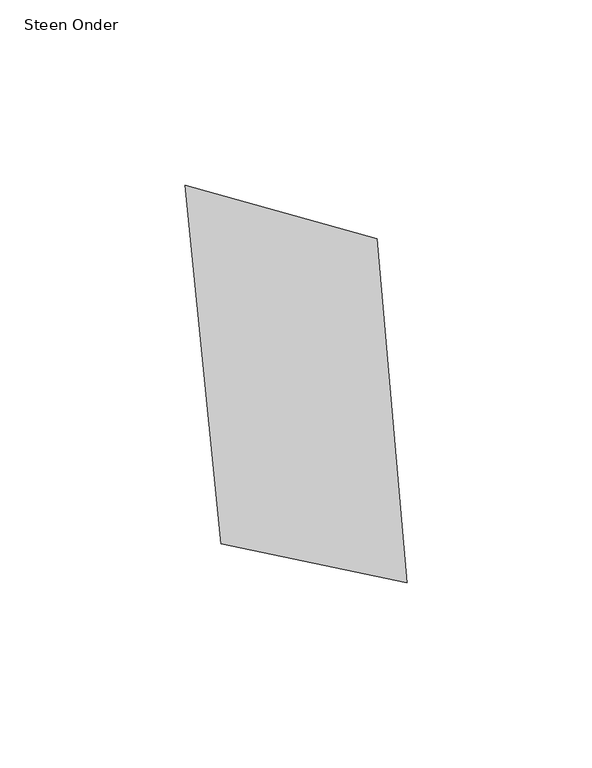
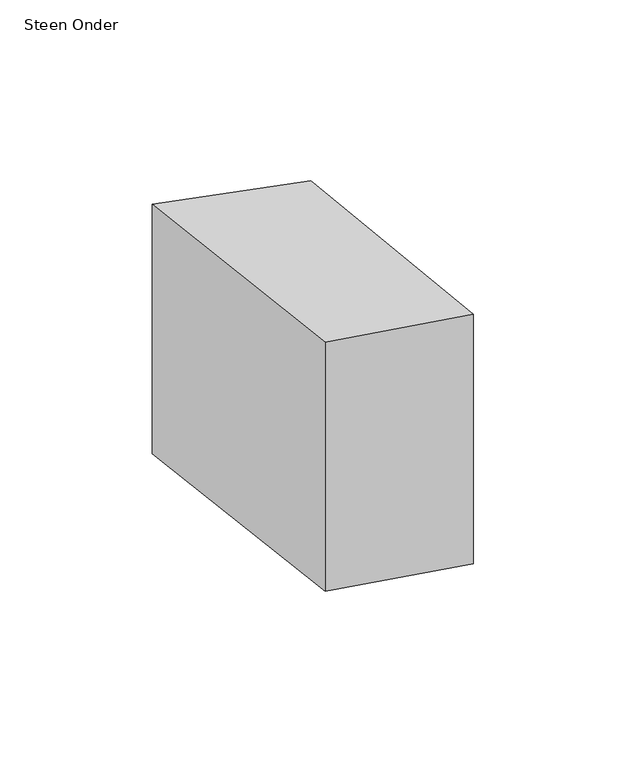
"""IFC4 building model written with IfcOpenShell, lengths in millimetres: proxy geometry, 00_GMA_steen_versie_4 : Steen Onder."""

import ifcopenshell
import ifcopenshell.guid

model = None  # the IFC model being written
_history = None  # IfcOwnerHistory: only IFC2X3 demands one
_inside = {}  # id of a spatial element -> (the spatial element, [elements in it])
_under = {}  # id of a project, library or spatial element -> (it, [spatial elements below it])
_declared = {}  # id of a project -> (the project, [libraries it declares])
_typed = {}  # id of a type object -> (the type object, [elements of that type])
_made_of = {}  # id of a material, layer set ... -> (it, [elements and type objects made of it])


def new_model(schema):
    """Start an empty IFC model of exactly this schema.

    Asked for "IFC4X3", IfcOpenShell would pick the latest addendum, in which some entities
    have other attributes; the version numbers below select the first issue.
    IFC2X3 requires an IfcOwnerHistory on every rooted entity: one is made here for all.
    """
    global model, _history
    if schema == "IFC4X3":
        model = ifcopenshell.file(schema_version=(4, 3, 0, 0))
    else:
        model = ifcopenshell.file(schema=schema)
    _inside.clear()
    _under.clear()
    _declared.clear()
    _typed.clear()
    _made_of.clear()
    _history = None
    if model.schema == "IFC2X3":
        org = make("IfcOrganization", Name="unknown")
        user = make(
            "IfcPersonAndOrganization",
            ThePerson=make("IfcPerson", FamilyName="unknown"),
            TheOrganization=org,
        )
        app = make(
            "IfcApplication",
            ApplicationDeveloper=org,
            Version="unknown",
            ApplicationFullName="unknown",
            ApplicationIdentifier="unknown",
        )
        _history = make(
            "IfcOwnerHistory",
            OwningUser=user,
            OwningApplication=app,
            ChangeAction="ADDED",
            CreationDate=0,
        )
    return model


def make(cls, **values):
    """One entity of the class cls with the attributes given. An attribute that is None is left unset."""
    return model.create_entity(
        cls, **{name: value for name, value in values.items() if value is not None}
    )


def rooted(cls, **values):
    """An entity with a GlobalId (a new one), such as an element, a storey or a relation."""
    return make(cls, GlobalId=ifcopenshell.guid.new(), OwnerHistory=_history, **values)


def si_unit(unit_type, name, prefix=None):
    """IfcSIUnit, for example si_unit("LENGTHUNIT", "METRE", prefix="MILLI")."""
    return make("IfcSIUnit", UnitType=unit_type, Prefix=prefix, Name=name)


def assignment(units):
    """IfcUnitAssignment: the units of a project."""
    return None if units is None else make("IfcUnitAssignment", Units=units)


def point(xyz):
    """IfcCartesianPoint."""
    return None if xyz is None else make("IfcCartesianPoint", Coordinates=xyz)


def direction(xyz):
    """IfcDirection."""
    return None if xyz is None else make("IfcDirection", DirectionRatios=xyz)


def frame(location, z_axis=None, x_axis=None):
    """IfcAxis2Placement3D, a coordinate frame: its origin and axes. An axis left out is left unset."""
    return make(
        "IfcAxis2Placement3D",
        Location=point(location),
        Axis=direction(z_axis),
        RefDirection=direction(x_axis),
    )


def origin():
    """The frame at (0, 0, 0) with its axes left unset."""
    return frame((0.0, 0.0, 0.0))


def origin_with_axes():
    """The frame at (0, 0, 0) with the z axis (0, 0, 1) and the x axis (1, 0, 0) written out."""
    return frame((0.0, 0.0, 0.0), z_axis=(0.0, 0.0, 1.0), x_axis=(1.0, 0.0, 0.0))


def place(relative_to, where):
    """IfcLocalPlacement: puts the frame where relative to a parent placement (None: the world)."""
    return make(
        "IfcLocalPlacement", PlacementRelTo=relative_to, RelativePlacement=where
    )


def context(
    kind, dimensions, precision=None, world=None, true_north=None, identifier=None
):
    """IfcGeometricRepresentationContext, for example the 3D "Model" context."""
    return make(
        "IfcGeometricRepresentationContext",
        ContextIdentifier=identifier,
        ContextType=kind,
        CoordinateSpaceDimension=dimensions,
        Precision=precision,
        WorldCoordinateSystem=world,
        TrueNorth=true_north,
    )


def project(units=None, contexts=None):
    """IfcProject with its units and contexts."""
    return rooted(
        "IfcProject",
        Name="project",
        RepresentationContexts=contexts,
        UnitsInContext=assignment(units),
    )


def spatial(cls, under=None, at=None, **own):
    """A site, building, storey or space (cls), placed at a placement, below another one or the project."""
    s = rooted(cls, ObjectPlacement=at, **own)
    if under is not None:
        _under.setdefault(under.id(), (under, []))[1].append(s)
    return s


def polyline(points):
    """IfcPolyline through the points."""
    return make("IfcPolyline", Points=[point(p) for p in points])


def outline(outer, holes=None, kind="AREA"):
    """IfcArbitraryClosedProfileDef: a profile drawn as a closed curve; with holes, ...WithVoids."""
    if holes is None:
        return make("IfcArbitraryClosedProfileDef", ProfileType=kind, OuterCurve=outer)
    return make(
        "IfcArbitraryProfileDefWithVoids",
        ProfileType=kind,
        OuterCurve=outer,
        InnerCurves=holes,
    )


def extrude(swept, where, along, depth):
    """IfcExtrudedAreaSolid: the profile swept, set in the frame where, extruded along a direction by depth."""
    return make(
        "IfcExtrudedAreaSolid",
        SweptArea=swept,
        Position=where,
        ExtrudedDirection=direction(along),
        Depth=depth,
    )


def shape(context_of_items, identifier, shape_type, items):
    """IfcShapeRepresentation: the items that make up one representation, for example the "Body"."""
    return make(
        "IfcShapeRepresentation",
        ContextOfItems=context_of_items,
        RepresentationIdentifier=identifier,
        RepresentationType=shape_type,
        Items=items,
    )


def source(mapping_origin, context_of_items, identifier, shape_type, items):
    """IfcRepresentationMap: a shape defined once, which mapped items show again and again."""
    return make(
        "IfcRepresentationMap",
        MappingOrigin=mapping_origin,
        MappedRepresentation=shape(context_of_items, identifier, shape_type, items),
    )


def transform(
    local_origin,
    x_axis=None,
    y_axis=None,
    z_axis=None,
    scale=None,
    scale2=None,
    scale3=None,
    uniform=True,
):
    """IfcCartesianTransformationOperator3D, or its non-uniform kind. x_axis, y_axis, z_axis: its Axis1, 2, 3."""
    if uniform:
        return make(
            "IfcCartesianTransformationOperator3D",
            Axis1=direction(x_axis),
            Axis2=direction(y_axis),
            LocalOrigin=point(local_origin),
            Scale=scale,
            Axis3=direction(z_axis),
        )
    return make(
        "IfcCartesianTransformationOperator3DnonUniform",
        Axis1=direction(x_axis),
        Axis2=direction(y_axis),
        LocalOrigin=point(local_origin),
        Scale=scale,
        Axis3=direction(z_axis),
        Scale2=scale2,
        Scale3=scale3,
    )


def mapped(mapping_source, mapping_target):
    """IfcMappedItem: shows the shape of a source again, moved by a transform."""
    return make(
        "IfcMappedItem", MappingSource=mapping_source, MappingTarget=mapping_target
    )


def made_of(thing, what):
    """Note that an element or type object is made of a material, layer set ...; save() writes the relation."""
    if what is not None:
        _made_of.setdefault(what.id(), (what, []))[1].append(thing)
    return thing


def element(
    cls,
    number,
    at=None,
    inside=None,
    cuts=None,
    type_object=None,
    material=None,
    context=None,
    identifier="Body",
    shape_type=None,
    held_by="IfcProductDefinitionShape",
    body=None,
    shapes=None,
    **own,
):
    """One element of the class cls, such as IfcWall. Its Tag is "e" and its number.

    at: its placement. inside: the storey or other place that contains it. cuts: it is an
    opening in that element (IfcRelVoidsElement). A single representation is given by context,
    identifier, shape_type and body (its items); several are given by shapes. held_by: the class
    of the entity that holds the representations. save() writes the other relations.
    """
    e = rooted(cls, Tag="e%d" % number, ObjectPlacement=at, **own)
    if body is not None:
        shapes = [shape(context, identifier, shape_type, body)]
    if shapes is not None:
        e.Representation = make(held_by, Representations=shapes)
    if inside is not None:
        _inside.setdefault(inside.id(), (inside, []))[1].append(e)
    if cuts is not None:
        rooted(
            "IfcRelVoidsElement", RelatingBuildingElement=cuts, RelatedOpeningElement=e
        )
    if type_object is not None:
        _typed.setdefault(type_object.id(), (type_object, []))[1].append(e)
    return made_of(e, material)


def aggregate(whole, parts):
    """IfcRelAggregates: a whole, such as a stair, and the parts it consists of."""
    return rooted("IfcRelAggregates", RelatingObject=whole, RelatedObjects=parts)


def save(model, path):
    """Write the relations noted so far, then the file.

    IfcRelAggregates (storeys below a building ...), IfcRelContainedInSpatialStructure (elements
    in a storey), IfcRelDefinesByType, IfcRelAssociatesMaterial and IfcRelDeclares: one each for
    every whole, place, type object, material and project.
    """
    for whole, parts in _under.values():
        aggregate(whole, parts)
    for where, things in _inside.values():
        rooted(
            "IfcRelContainedInSpatialStructure",
            RelatedElements=things,
            RelatingStructure=where,
        )
    for kind, things in _typed.values():
        rooted("IfcRelDefinesByType", RelatedObjects=things, RelatingType=kind)
    for what, things in _made_of.values():
        rooted("IfcRelAssociatesMaterial", RelatedObjects=things, RelatingMaterial=what)
    for by, libraries in _declared.values():
        rooted("IfcRelDeclares", RelatingContext=by, RelatedDefinitions=libraries)
    model.write(path)


def steen_onder_f9fddc1d(model_context):
    return source(origin(), model_context, "Body", "SweptSolid", [
        extrude(outline(polyline([(96.9265874, 113.8378583), (104.9232628, 20.8363381), (54.7198036, 31.3553281), (44.9541257, 128.2804905), (96.9265874, 113.8378583)])), origin_with_axes(), (0.0, 0.0, 1.0), 100.0),
    ])


if __name__ == "__main__":
    model = new_model("IFC4")
    model_context = context("Model", 3, world=origin())
    ifc_project = project(units=[si_unit("LENGTHUNIT", "METRE", prefix="MILLI")], contexts=[model_context])
    site = spatial("IfcSite", under=ifc_project)
    building = spatial("IfcBuilding", under=site)
    placement = place(None, origin())
    steen_onder_shape = steen_onder_f9fddc1d(model_context)
    element("IfcBuildingElementProxy", 1, Name="00_GMA_steen_versie_4 : Steen Onder", ObjectType="00_GMA_steen_versie_4 : Steen Onder", at=placement, inside=building, context=model_context, shape_type="MappedRepresentation", body=[
        mapped(steen_onder_shape, transform((0.0, 0.0, 0.0), x_axis=(1.0, 0.0, 0.0), y_axis=(0.0, 1.0, 0.0), z_axis=(0.0, 0.0, 1.0))),
    ])
    save(model, "model.ifc")

# Revit data of these elements
# Type "00_GMA_steen_versie_4 : Steen Onder"
#   StootVoegHalfBoven [instance default] = 5 mm
#   StootVoegHalf [instance default] = 5 mm
#   StootVoegBreedteOnder = 10 mm
#   StootVoegBreedteBoven = 10 mm
#   Steendikte = 100 mm
#   LintVoegOnderHalf = 0 mm
#   LintVoegOnder = 0 mm
#   LintVoegBovenHalf = 5 mm
#   LintVoegBoven = 10 mm
#   materiaal = none
#   MateriaalVoeg = none
#   Default Elevation = 0
